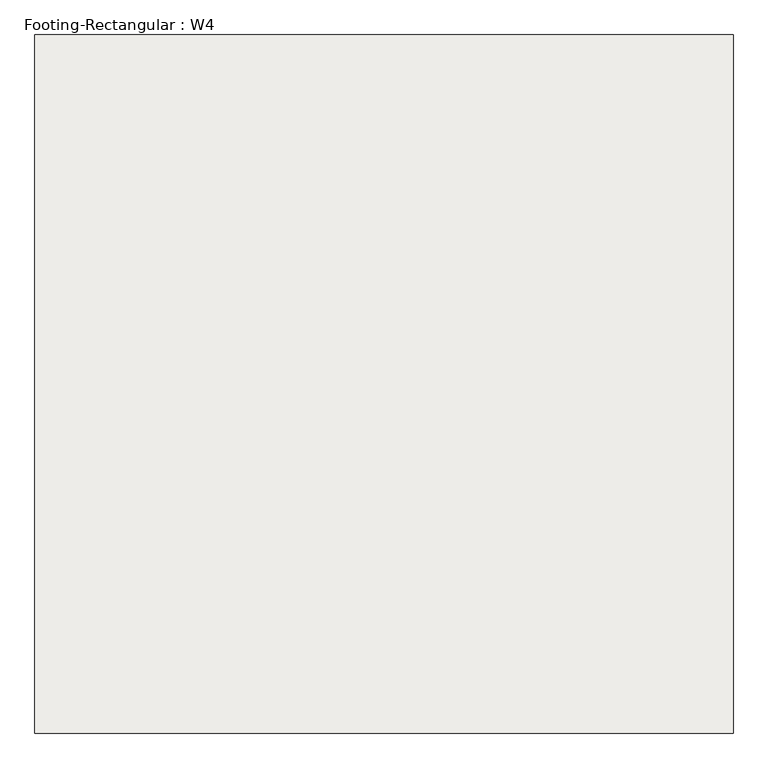
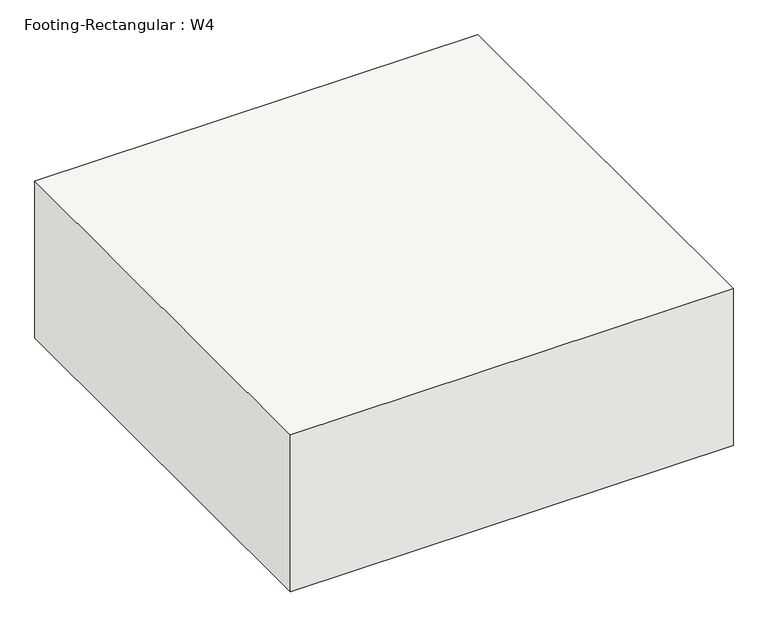
"""IFC4 building model written with IfcOpenShell, lengths in millimetres: slab geometry, Footing-Rectangular : W4."""

from ifc_helpers import new_model, si_unit, frame, origin, place, context, project, spatial, polyline, outline, extrude, source, transform, mapped, element, save


def footing_rectangular_w4_ae0d545e(model_context):
    return source(origin(), model_context, "Body", "SweptSolid", [
        extrude(outline(polyline([(609.6, 609.6), (609.6, -609.6), (-609.6, -609.6), (-609.6, 609.6), (609.6, 609.6)])), frame((0.0, 0.0, -457.2), z_axis=(0.0, 0.0, 1.0), x_axis=(1.0, 0.0, 0.0)), (0.0, 0.0, 1.0), 457.2),
    ])


if __name__ == "__main__":
    model = new_model("IFC4")
    model_context = context("Model", 3, world=origin())
    ifc_project = project(units=[si_unit("LENGTHUNIT", "METRE", prefix="MILLI")], contexts=[model_context])
    site = spatial("IfcSite", under=ifc_project)
    building = spatial("IfcBuilding", under=site)
    placement = place(None, origin())
    footing_rectangular_w4_shape = footing_rectangular_w4_ae0d545e(model_context)
    element("IfcSlab", 1, ObjectType="Footing-Rectangular : W4", at=placement, inside=building, context=model_context, shape_type="MappedRepresentation", body=[
        mapped(footing_rectangular_w4_shape, transform((0.0, 0.0, 0.0), x_axis=(1.0, 0.0, 0.0), y_axis=(0.0, 1.0, 0.0), z_axis=(0.0, 0.0, 1.0))),
    ])
    save(model, "model.ifc")

# Revit data of these elements
# Type "Footing-Rectangular : W4"
#   Assembly Code = "A1010100"
#   Width = 4' - 0"
#   Length = 4' - 0"
#   Foundation Thickness = 1' - 6"
#   Structural Material [instance default] = Concrete, Cast-in-Place gray
# Element 1 (IfcSlab, "Footing-Rectangular : W4")
#   Materials on its faces: "Concrete, Cast-in-Place gray"
# Materials
#   "Concrete, Cast-in-Place gray": class "Concrete", colour RGB 192 192 192, transparency 0, Description = "Cast-in-place concrete", Cost = 0
